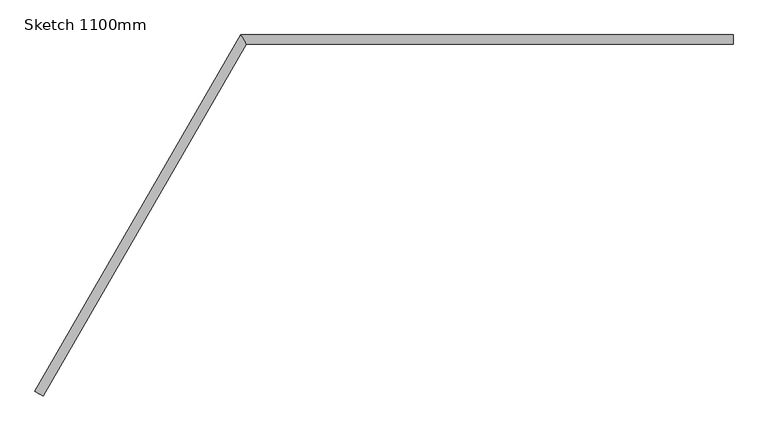
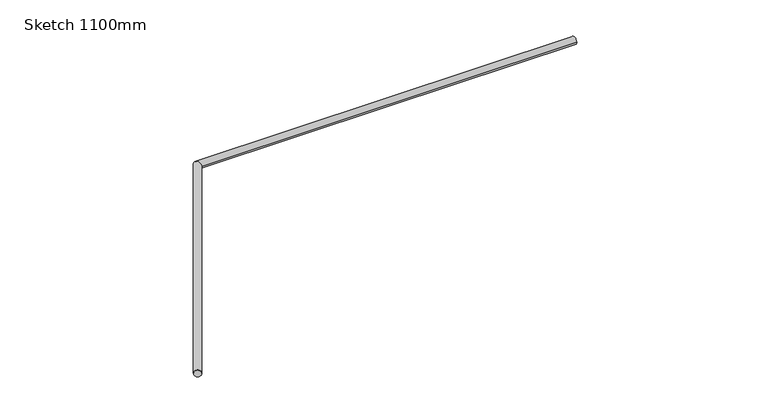
"""IFC4 building model written with IfcOpenShell, lengths in millimetres: railing geometry, Sketch 1100mm."""

import ifcopenshell
import ifcopenshell.guid

model = None  # the IFC model being written
_history = None  # IfcOwnerHistory: only IFC2X3 demands one
_inside = {}  # id of a spatial element -> (the spatial element, [elements in it])
_under = {}  # id of a project, library or spatial element -> (it, [spatial elements below it])
_declared = {}  # id of a project -> (the project, [libraries it declares])
_typed = {}  # id of a type object -> (the type object, [elements of that type])
_made_of = {}  # id of a material, layer set ... -> (it, [elements and type objects made of it])


def new_model(schema):
    """Start an empty IFC model of exactly this schema.

    Asked for "IFC4X3", IfcOpenShell would pick the latest addendum, in which some entities
    have other attributes; the version numbers below select the first issue.
    IFC2X3 requires an IfcOwnerHistory on every rooted entity: one is made here for all.
    """
    global model, _history
    if schema == "IFC4X3":
        model = ifcopenshell.file(schema_version=(4, 3, 0, 0))
    else:
        model = ifcopenshell.file(schema=schema)
    _inside.clear()
    _under.clear()
    _declared.clear()
    _typed.clear()
    _made_of.clear()
    _history = None
    if model.schema == "IFC2X3":
        org = make("IfcOrganization", Name="unknown")
        user = make(
            "IfcPersonAndOrganization",
            ThePerson=make("IfcPerson", FamilyName="unknown"),
            TheOrganization=org,
        )
        app = make(
            "IfcApplication",
            ApplicationDeveloper=org,
            Version="unknown",
            ApplicationFullName="unknown",
            ApplicationIdentifier="unknown",
        )
        _history = make(
            "IfcOwnerHistory",
            OwningUser=user,
            OwningApplication=app,
            ChangeAction="ADDED",
            CreationDate=0,
        )
    return model


def make(cls, **values):
    """One entity of the class cls with the attributes given. An attribute that is None is left unset."""
    return model.create_entity(
        cls, **{name: value for name, value in values.items() if value is not None}
    )


def rooted(cls, **values):
    """An entity with a GlobalId (a new one), such as an element, a storey or a relation."""
    return make(cls, GlobalId=ifcopenshell.guid.new(), OwnerHistory=_history, **values)


def si_unit(unit_type, name, prefix=None):
    """IfcSIUnit, for example si_unit("LENGTHUNIT", "METRE", prefix="MILLI")."""
    return make("IfcSIUnit", UnitType=unit_type, Prefix=prefix, Name=name)


def assignment(units):
    """IfcUnitAssignment: the units of a project."""
    return None if units is None else make("IfcUnitAssignment", Units=units)


def point(xyz):
    """IfcCartesianPoint."""
    return None if xyz is None else make("IfcCartesianPoint", Coordinates=xyz)


def direction(xyz):
    """IfcDirection."""
    return None if xyz is None else make("IfcDirection", DirectionRatios=xyz)


def frame(location, z_axis=None, x_axis=None):
    """IfcAxis2Placement3D, a coordinate frame: its origin and axes. An axis left out is left unset."""
    return make(
        "IfcAxis2Placement3D",
        Location=point(location),
        Axis=direction(z_axis),
        RefDirection=direction(x_axis),
    )


def origin():
    """The frame at (0, 0, 0) with its axes left unset."""
    return frame((0.0, 0.0, 0.0))


def place(relative_to, where):
    """IfcLocalPlacement: puts the frame where relative to a parent placement (None: the world)."""
    return make(
        "IfcLocalPlacement", PlacementRelTo=relative_to, RelativePlacement=where
    )


def context(
    kind, dimensions, precision=None, world=None, true_north=None, identifier=None
):
    """IfcGeometricRepresentationContext, for example the 3D "Model" context."""
    return make(
        "IfcGeometricRepresentationContext",
        ContextIdentifier=identifier,
        ContextType=kind,
        CoordinateSpaceDimension=dimensions,
        Precision=precision,
        WorldCoordinateSystem=world,
        TrueNorth=true_north,
    )


def project(units=None, contexts=None):
    """IfcProject with its units and contexts."""
    return rooted(
        "IfcProject",
        Name="project",
        RepresentationContexts=contexts,
        UnitsInContext=assignment(units),
    )


def spatial(cls, under=None, at=None, **own):
    """A site, building, storey or space (cls), placed at a placement, below another one or the project."""
    s = rooted(cls, ObjectPlacement=at, **own)
    if under is not None:
        _under.setdefault(under.id(), (under, []))[1].append(s)
    return s


def circle_curve(where, radius):
    """IfcCircle in the frame where."""
    return make("IfcCircle", Position=where, Radius=radius)


def ellipse_curve(where, semi_axis1, semi_axis2):
    """IfcEllipse in the frame where."""
    return make(
        "IfcEllipse", Position=where, SemiAxis1=semi_axis1, SemiAxis2=semi_axis2
    )


def shape(context_of_items, identifier, shape_type, items):
    """IfcShapeRepresentation: the items that make up one representation, for example the "Body"."""
    return make(
        "IfcShapeRepresentation",
        ContextOfItems=context_of_items,
        RepresentationIdentifier=identifier,
        RepresentationType=shape_type,
        Items=items,
    )


def source(mapping_origin, context_of_items, identifier, shape_type, items):
    """IfcRepresentationMap: a shape defined once, which mapped items show again and again."""
    return make(
        "IfcRepresentationMap",
        MappingOrigin=mapping_origin,
        MappedRepresentation=shape(context_of_items, identifier, shape_type, items),
    )


def transform(
    local_origin,
    x_axis=None,
    y_axis=None,
    z_axis=None,
    scale=None,
    scale2=None,
    scale3=None,
    uniform=True,
):
    """IfcCartesianTransformationOperator3D, or its non-uniform kind. x_axis, y_axis, z_axis: its Axis1, 2, 3."""
    if uniform:
        return make(
            "IfcCartesianTransformationOperator3D",
            Axis1=direction(x_axis),
            Axis2=direction(y_axis),
            LocalOrigin=point(local_origin),
            Scale=scale,
            Axis3=direction(z_axis),
        )
    return make(
        "IfcCartesianTransformationOperator3DnonUniform",
        Axis1=direction(x_axis),
        Axis2=direction(y_axis),
        LocalOrigin=point(local_origin),
        Scale=scale,
        Axis3=direction(z_axis),
        Scale2=scale2,
        Scale3=scale3,
    )


def mapped(mapping_source, mapping_target):
    """IfcMappedItem: shows the shape of a source again, moved by a transform."""
    return make(
        "IfcMappedItem", MappingSource=mapping_source, MappingTarget=mapping_target
    )


def made_of(thing, what):
    """Note that an element or type object is made of a material, layer set ...; save() writes the relation."""
    if what is not None:
        _made_of.setdefault(what.id(), (what, []))[1].append(thing)
    return thing


def element(
    cls,
    number,
    at=None,
    inside=None,
    cuts=None,
    type_object=None,
    material=None,
    context=None,
    identifier="Body",
    shape_type=None,
    held_by="IfcProductDefinitionShape",
    body=None,
    shapes=None,
    **own,
):
    """One element of the class cls, such as IfcWall. Its Tag is "e" and its number.

    at: its placement. inside: the storey or other place that contains it. cuts: it is an
    opening in that element (IfcRelVoidsElement). A single representation is given by context,
    identifier, shape_type and body (its items); several are given by shapes. held_by: the class
    of the entity that holds the representations. save() writes the other relations.
    """
    e = rooted(cls, Tag="e%d" % number, ObjectPlacement=at, **own)
    if body is not None:
        shapes = [shape(context, identifier, shape_type, body)]
    if shapes is not None:
        e.Representation = make(held_by, Representations=shapes)
    if inside is not None:
        _inside.setdefault(inside.id(), (inside, []))[1].append(e)
    if cuts is not None:
        rooted(
            "IfcRelVoidsElement", RelatingBuildingElement=cuts, RelatedOpeningElement=e
        )
    if type_object is not None:
        _typed.setdefault(type_object.id(), (type_object, []))[1].append(e)
    return made_of(e, material)


def aggregate(whole, parts):
    """IfcRelAggregates: a whole, such as a stair, and the parts it consists of."""
    return rooted("IfcRelAggregates", RelatingObject=whole, RelatedObjects=parts)


def save(model, path):
    """Write the relations noted so far, then the file.

    IfcRelAggregates (storeys below a building ...), IfcRelContainedInSpatialStructure (elements
    in a storey), IfcRelDefinesByType, IfcRelAssociatesMaterial and IfcRelDeclares: one each for
    every whole, place, type object, material and project.
    """
    for whole, parts in _under.values():
        aggregate(whole, parts)
    for where, things in _inside.values():
        rooted(
            "IfcRelContainedInSpatialStructure",
            RelatedElements=things,
            RelatingStructure=where,
        )
    for kind, things in _typed.values():
        rooted("IfcRelDefinesByType", RelatedObjects=things, RelatingType=kind)
    for what, things in _made_of.values():
        rooted("IfcRelAssociatesMaterial", RelatedObjects=things, RelatingMaterial=what)
    for by, libraries in _declared.values():
        rooted("IfcRelDeclares", RelatingContext=by, RelatedDefinitions=libraries)
    model.write(path)


def plane_surface(at):
    """IfcPlane: the flat surface through the origin of the frame at, square to its z axis."""
    return make("IfcPlane", Position=at)


def cylinder_surface(at, radius):
    """IfcCylindricalSurface: all points at the distance radius from the z axis of the frame at."""
    return make("IfcCylindricalSurface", Position=at, Radius=radius)


def advanced_brep(points, edges, surfaces, faces):
    """IfcAdvancedBrep: a solid bounded by faces that lie on surfaces and meet in shared edges.

    An edge is (start, end): straight between two places in points (the first is 0);
    or (start, end, curve); or (start, end, curve, False) where it runs against its curve.
    A face is (place in surfaces, loops), or (place, loops, False) where it looks against
    its surface's normal. A loop lists edges by number (the first is 1), with a minus sign
    where the edge is run from its end to its start. The first loop is the outer one.
    """
    corners = [point(p) for p in points]
    vertices = [make("IfcVertexPoint", VertexGeometry=c) for c in corners]
    made = []
    for start, end, *more in edges:
        made.append(
            make(
                "IfcEdgeCurve",
                EdgeStart=vertices[start],
                EdgeEnd=vertices[end],
                EdgeGeometry=more[0] if more else make("IfcPolyline", Points=[corners[start], corners[end]]),
                SameSense=more[1] if len(more) > 1 else True,
            )
        )
    hull = []
    for where, loops, *sense in faces:
        bounds = []
        for j, loop in enumerate(loops):
            ring = [make("IfcOrientedEdge", EdgeElement=made[abs(k) - 1], Orientation=k > 0) for k in loop]
            bounds.append(
                make(
                    "IfcFaceOuterBound" if j == 0 else "IfcFaceBound",
                    Bound=make("IfcEdgeLoop", EdgeList=ring),
                    Orientation=True,
                )
            )
        hull.append(make("IfcAdvancedFace", Bounds=bounds, FaceSurface=surfaces[where], SameSense=sense[0] if sense else True))
    return make("IfcAdvancedBrep", Outer=make("IfcClosedShell", CfsFaces=hull))


def sketch_1100mm_c51240ad(model_context):
    return source(origin(), model_context, "Body", "AdvancedBrep", [
        advanced_brep(
        [(3000.0, 60.0, 4280.0), (2965.3589838, 80.0, 4280.0), (3842.931393, 1600.0, 4280.0), (3866.0254038, 1560.0, 4280.0), (5940.0, 1560.0, 4280.0), (5940.0, 1600.0, 4280.0)],
        [
            (0, 1, circle_curve(frame((2982.6794919, 70.0, 4280.0), z_axis=(-0.5000000000000013, -0.8660254037844379, 0.0), x_axis=(-0.8660254037844379, 0.5000000000000013, 0.0)), 20.0)),
            (1, 0, circle_curve(frame((2982.6794919, 70.0, 4280.0), z_axis=(-0.5000000000000013, -0.8660254037844379, 0.0), x_axis=(-0.8660254037844379, 0.5000000000000013, 0.0)), 20.0)),
            (1, 2),
            (2, 3, ellipse_curve(frame((3854.4783984, 1580.0, 4280.0), z_axis=(-0.8660254037844398, -0.49999999999999795, 0.0), x_axis=(0.4999999999999979, -0.8660254037844398, 0.0)), 23.0940108, 20.0)),
            (3, 0),
            (3, 2, ellipse_curve(frame((3854.4783984, 1580.0, 4280.0), z_axis=(-0.8660254037844398, -0.49999999999999795, 0.0), x_axis=(0.4999999999999979, -0.8660254037844398, 0.0)), 23.0940108, 20.0)),
            (4, 5, circle_curve(frame((5940.0, 1580.0, 4280.0), z_axis=(1.0, 0.0, 0.0), x_axis=(0.0, 1.0, 0.0)), 20.0)),
            (5, 4, circle_curve(frame((5940.0, 1580.0, 4280.0), z_axis=(1.0, 0.0, 0.0), x_axis=(0.0, 1.0, 0.0)), 20.0)),
            (2, 5),
            (4, 3),
        ],
        [
            plane_surface(frame((2982.6794919, 70.0, 4300.0), z_axis=(-0.5000000000000014, -0.8660254037844379, 0.0), x_axis=(0.8660254037844379, -0.5000000000000014, 0.0))),
            cylinder_surface(frame((2982.6794919, 70.0, 4280.0), z_axis=(-0.5000000000000013, -0.8660254037844379, 0.0), x_axis=(-0.8660254037844379, 0.5000000000000013, 0.0)), 20.0),
            plane_surface(frame((5940.0, 1580.0, 4300.0), z_axis=(1.0, 0.0, 0.0), x_axis=(0.0, 1.0, 0.0))),
            cylinder_surface(frame((3854.4783984, 1580.0, 4280.0), z_axis=(-1.0, 0.0, 0.0), x_axis=(0.0, 1.0, 0.0)), 20.0),
        ],
        [
            (0, [[1, 2]]),
            (1, [[-2, 3, 4, 5]]),
            (1, [[-1, -5, 6, -3]]),
            (2, [[7, 8]]),
            (3, [[-4, 9, -7, 10]]),
            (3, [[-6, -10, -8, -9]]),
        ],
    ),
    ])


if __name__ == "__main__":
    model = new_model("IFC4")
    model_context = context("Model", 3, world=origin())
    ifc_project = project(units=[si_unit("LENGTHUNIT", "METRE", prefix="MILLI")], contexts=[model_context])
    site = spatial("IfcSite", under=ifc_project)
    building = spatial("IfcBuilding", under=site)
    placement = place(None, origin())
    sketch_1100mm_shape = sketch_1100mm_c51240ad(model_context)
    element("IfcRailing", 1, ObjectType="Sketch 1100mm", at=placement, inside=building, context=model_context, shape_type="MappedRepresentation", body=[
        mapped(sketch_1100mm_shape, transform((0.0, 0.0, 0.0), x_axis=(1.0, 0.0, 0.0), y_axis=(0.0, 1.0, 0.0), z_axis=(0.0, 0.0, 1.0))),
    ])
    save(model, "model.ifc")

# Revit data of these elements
# Element 1 (IfcRailing, "Sketch 1100mm")
#   Materials on its faces: "Default Railings (Interior/Exterior)"
# Materials
#   "Default Railings (Interior/Exterior)": class "Generic", colour RGB 205 205 205, transparency 0, Description = "Udefineret gelænder materiale", Cost = 0
